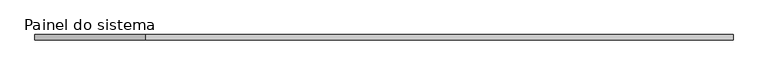
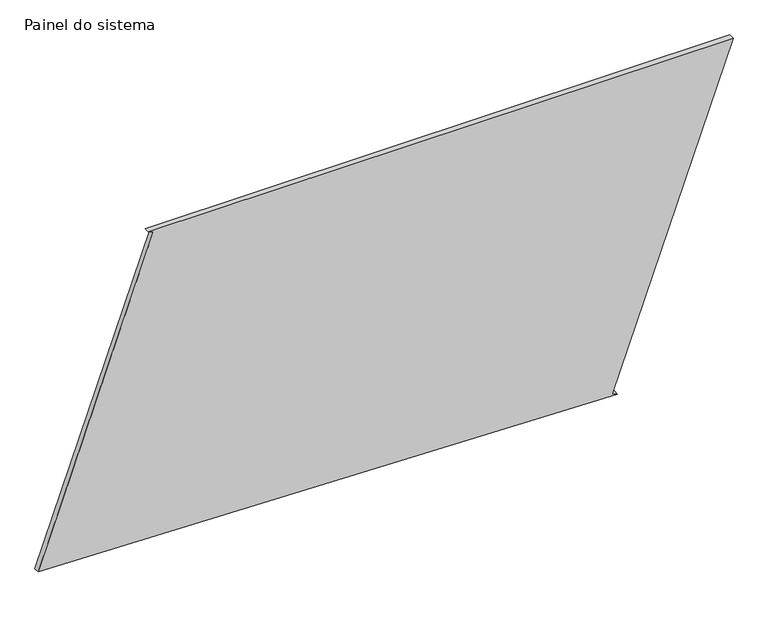
"""IFC4 building model written with IfcOpenShell, lengths in millimetres: plate geometry, Painel do sistema : Envidraçado."""

import ifcopenshell
import ifcopenshell.guid

model = None  # the IFC model being written
_history = None  # IfcOwnerHistory: only IFC2X3 demands one
_inside = {}  # id of a spatial element -> (the spatial element, [elements in it])
_under = {}  # id of a project, library or spatial element -> (it, [spatial elements below it])
_declared = {}  # id of a project -> (the project, [libraries it declares])
_typed = {}  # id of a type object -> (the type object, [elements of that type])
_made_of = {}  # id of a material, layer set ... -> (it, [elements and type objects made of it])


def new_model(schema):
    """Start an empty IFC model of exactly this schema.

    Asked for "IFC4X3", IfcOpenShell would pick the latest addendum, in which some entities
    have other attributes; the version numbers below select the first issue.
    IFC2X3 requires an IfcOwnerHistory on every rooted entity: one is made here for all.
    """
    global model, _history
    if schema == "IFC4X3":
        model = ifcopenshell.file(schema_version=(4, 3, 0, 0))
    else:
        model = ifcopenshell.file(schema=schema)
    _inside.clear()
    _under.clear()
    _declared.clear()
    _typed.clear()
    _made_of.clear()
    _history = None
    if model.schema == "IFC2X3":
        org = make("IfcOrganization", Name="unknown")
        user = make(
            "IfcPersonAndOrganization",
            ThePerson=make("IfcPerson", FamilyName="unknown"),
            TheOrganization=org,
        )
        app = make(
            "IfcApplication",
            ApplicationDeveloper=org,
            Version="unknown",
            ApplicationFullName="unknown",
            ApplicationIdentifier="unknown",
        )
        _history = make(
            "IfcOwnerHistory",
            OwningUser=user,
            OwningApplication=app,
            ChangeAction="ADDED",
            CreationDate=0,
        )
    return model


def make(cls, **values):
    """One entity of the class cls with the attributes given. An attribute that is None is left unset."""
    return model.create_entity(
        cls, **{name: value for name, value in values.items() if value is not None}
    )


def rooted(cls, **values):
    """An entity with a GlobalId (a new one), such as an element, a storey or a relation."""
    return make(cls, GlobalId=ifcopenshell.guid.new(), OwnerHistory=_history, **values)


def si_unit(unit_type, name, prefix=None):
    """IfcSIUnit, for example si_unit("LENGTHUNIT", "METRE", prefix="MILLI")."""
    return make("IfcSIUnit", UnitType=unit_type, Prefix=prefix, Name=name)


def assignment(units):
    """IfcUnitAssignment: the units of a project."""
    return None if units is None else make("IfcUnitAssignment", Units=units)


def point(xyz):
    """IfcCartesianPoint."""
    return None if xyz is None else make("IfcCartesianPoint", Coordinates=xyz)


def direction(xyz):
    """IfcDirection."""
    return None if xyz is None else make("IfcDirection", DirectionRatios=xyz)


def frame(location, z_axis=None, x_axis=None):
    """IfcAxis2Placement3D, a coordinate frame: its origin and axes. An axis left out is left unset."""
    return make(
        "IfcAxis2Placement3D",
        Location=point(location),
        Axis=direction(z_axis),
        RefDirection=direction(x_axis),
    )


def origin():
    """The frame at (0, 0, 0) with its axes left unset."""
    return frame((0.0, 0.0, 0.0))


def place(relative_to, where):
    """IfcLocalPlacement: puts the frame where relative to a parent placement (None: the world)."""
    return make(
        "IfcLocalPlacement", PlacementRelTo=relative_to, RelativePlacement=where
    )


def context(
    kind, dimensions, precision=None, world=None, true_north=None, identifier=None
):
    """IfcGeometricRepresentationContext, for example the 3D "Model" context."""
    return make(
        "IfcGeometricRepresentationContext",
        ContextIdentifier=identifier,
        ContextType=kind,
        CoordinateSpaceDimension=dimensions,
        Precision=precision,
        WorldCoordinateSystem=world,
        TrueNorth=true_north,
    )


def project(units=None, contexts=None):
    """IfcProject with its units and contexts."""
    return rooted(
        "IfcProject",
        Name="project",
        RepresentationContexts=contexts,
        UnitsInContext=assignment(units),
    )


def spatial(cls, under=None, at=None, **own):
    """A site, building, storey or space (cls), placed at a placement, below another one or the project."""
    s = rooted(cls, ObjectPlacement=at, **own)
    if under is not None:
        _under.setdefault(under.id(), (under, []))[1].append(s)
    return s


def polyline(points):
    """IfcPolyline through the points."""
    return make("IfcPolyline", Points=[point(p) for p in points])


def outline(outer, holes=None, kind="AREA"):
    """IfcArbitraryClosedProfileDef: a profile drawn as a closed curve; with holes, ...WithVoids."""
    if holes is None:
        return make("IfcArbitraryClosedProfileDef", ProfileType=kind, OuterCurve=outer)
    return make(
        "IfcArbitraryProfileDefWithVoids",
        ProfileType=kind,
        OuterCurve=outer,
        InnerCurves=holes,
    )


def extrude(swept, where, along, depth):
    """IfcExtrudedAreaSolid: the profile swept, set in the frame where, extruded along a direction by depth."""
    return make(
        "IfcExtrudedAreaSolid",
        SweptArea=swept,
        Position=where,
        ExtrudedDirection=direction(along),
        Depth=depth,
    )


def shape(context_of_items, identifier, shape_type, items):
    """IfcShapeRepresentation: the items that make up one representation, for example the "Body"."""
    return make(
        "IfcShapeRepresentation",
        ContextOfItems=context_of_items,
        RepresentationIdentifier=identifier,
        RepresentationType=shape_type,
        Items=items,
    )


def source(mapping_origin, context_of_items, identifier, shape_type, items):
    """IfcRepresentationMap: a shape defined once, which mapped items show again and again."""
    return make(
        "IfcRepresentationMap",
        MappingOrigin=mapping_origin,
        MappedRepresentation=shape(context_of_items, identifier, shape_type, items),
    )


def transform(
    local_origin,
    x_axis=None,
    y_axis=None,
    z_axis=None,
    scale=None,
    scale2=None,
    scale3=None,
    uniform=True,
):
    """IfcCartesianTransformationOperator3D, or its non-uniform kind. x_axis, y_axis, z_axis: its Axis1, 2, 3."""
    if uniform:
        return make(
            "IfcCartesianTransformationOperator3D",
            Axis1=direction(x_axis),
            Axis2=direction(y_axis),
            LocalOrigin=point(local_origin),
            Scale=scale,
            Axis3=direction(z_axis),
        )
    return make(
        "IfcCartesianTransformationOperator3DnonUniform",
        Axis1=direction(x_axis),
        Axis2=direction(y_axis),
        LocalOrigin=point(local_origin),
        Scale=scale,
        Axis3=direction(z_axis),
        Scale2=scale2,
        Scale3=scale3,
    )


def mapped(mapping_source, mapping_target):
    """IfcMappedItem: shows the shape of a source again, moved by a transform."""
    return make(
        "IfcMappedItem", MappingSource=mapping_source, MappingTarget=mapping_target
    )


def made_of(thing, what):
    """Note that an element or type object is made of a material, layer set ...; save() writes the relation."""
    if what is not None:
        _made_of.setdefault(what.id(), (what, []))[1].append(thing)
    return thing


def element(
    cls,
    number,
    at=None,
    inside=None,
    cuts=None,
    type_object=None,
    material=None,
    context=None,
    identifier="Body",
    shape_type=None,
    held_by="IfcProductDefinitionShape",
    body=None,
    shapes=None,
    **own,
):
    """One element of the class cls, such as IfcWall. Its Tag is "e" and its number.

    at: its placement. inside: the storey or other place that contains it. cuts: it is an
    opening in that element (IfcRelVoidsElement). A single representation is given by context,
    identifier, shape_type and body (its items); several are given by shapes. held_by: the class
    of the entity that holds the representations. save() writes the other relations.
    """
    e = rooted(cls, Tag="e%d" % number, ObjectPlacement=at, **own)
    if body is not None:
        shapes = [shape(context, identifier, shape_type, body)]
    if shapes is not None:
        e.Representation = make(held_by, Representations=shapes)
    if inside is not None:
        _inside.setdefault(inside.id(), (inside, []))[1].append(e)
    if cuts is not None:
        rooted(
            "IfcRelVoidsElement", RelatingBuildingElement=cuts, RelatedOpeningElement=e
        )
    if type_object is not None:
        _typed.setdefault(type_object.id(), (type_object, []))[1].append(e)
    return made_of(e, material)


def aggregate(whole, parts):
    """IfcRelAggregates: a whole, such as a stair, and the parts it consists of."""
    return rooted("IfcRelAggregates", RelatingObject=whole, RelatedObjects=parts)


def save(model, path):
    """Write the relations noted so far, then the file.

    IfcRelAggregates (storeys below a building ...), IfcRelContainedInSpatialStructure (elements
    in a storey), IfcRelDefinesByType, IfcRelAssociatesMaterial and IfcRelDeclares: one each for
    every whole, place, type object, material and project.
    """
    for whole, parts in _under.values():
        aggregate(whole, parts)
    for where, things in _inside.values():
        rooted(
            "IfcRelContainedInSpatialStructure",
            RelatedElements=things,
            RelatingStructure=where,
        )
    for kind, things in _typed.values():
        rooted("IfcRelDefinesByType", RelatedObjects=things, RelatingType=kind)
    for what, things in _made_of.values():
        rooted("IfcRelAssociatesMaterial", RelatedObjects=things, RelatingMaterial=what)
    for by, libraries in _declared.values():
        rooted("IfcRelDeclares", RelatingContext=by, RelatedDefinitions=libraries)
    model.write(path)


def painel_do_sistema_da6d2208(model_context):
    return source(origin(), model_context, "Body", "SweptSolid", [
        extrude(outline(polyline([(0.0, 1073.8736594), (8.505028, 1050.3648419), (1556.253693, 1610.3098819), (1556.253693, -1098.9171366), (1547.748665, -1075.4083191), (69.22288, -1610.3098819), (0.0, 1073.8736594)])), frame((0.0, 24.5, 0.0), z_axis=(0.0, 1.0, 0.0), x_axis=(0.0, 0.0, 1.0)), (0.0, 0.0, 1.0), 25.0),
    ])


if __name__ == "__main__":
    model = new_model("IFC4")
    model_context = context("Model", 3, world=origin())
    ifc_project = project(units=[si_unit("LENGTHUNIT", "METRE", prefix="MILLI")], contexts=[model_context])
    site = spatial("IfcSite", under=ifc_project)
    building = spatial("IfcBuilding", under=site)
    placement = place(None, origin())
    painel_do_sistema_shape = painel_do_sistema_da6d2208(model_context)
    element("IfcPlate", 1, ObjectType="Painel do sistema : Envidraçado", at=placement, inside=building, context=model_context, shape_type="MappedRepresentation", body=[
        mapped(painel_do_sistema_shape, transform((0.0, 0.0, 0.0), x_axis=(1.0, 0.0, 0.0), y_axis=(0.0, 1.0, 0.0), z_axis=(0.0, 0.0, 1.0))),
    ])
    save(model, "model.ifc")

# Revit data of these elements
# Type "Painel do sistema : Envidraçado"
#   Construction Type Id = "GSP4R"
#   Analytic Construction = "Vidraça única Pilkington 1/8 pol"
#   Visual Light Transmittance = 0.9
#   Solar Heat Gain Coefficient = 0.86
#   Heat Transfer Coefficient (U) = 6.7069 W/(m²·K)
# Element 1 (IfcPlate, "Painel do sistema : Envidraçado")
#   Materials on its faces: "Vidro"
# Materials
#   "Vidro": class "Vidro", colour RGB 0 128 192, transparency 0.9, Description = "Vidro de sílica", Cost = 0
